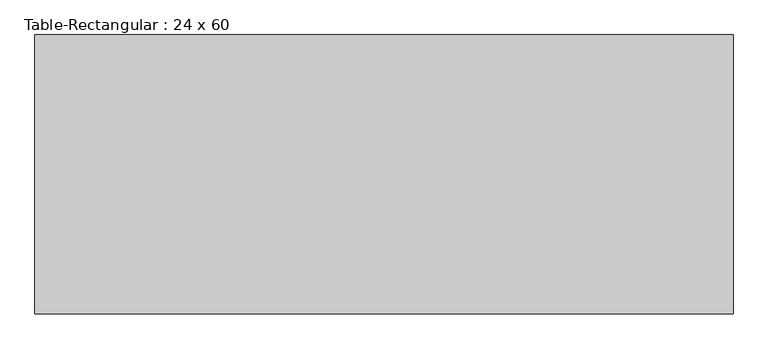
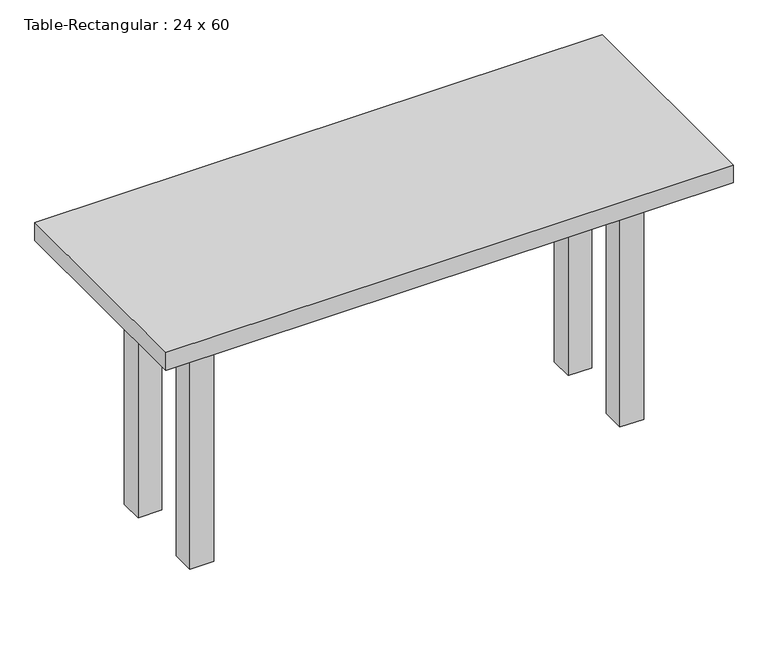
"""IFC4 building model written with IfcOpenShell, lengths in millimetres: furniture geometry, Table-Rectangular : 24 x 60."""

from ifc_helpers import new_model, si_unit, frame, origin, origin_with_axes, place, context, project, spatial, polyline, outline, extrude, source, transform, mapped, element, save


def table_rectangular_24_x_60_3e3a90ab(model_context):
    return source(origin(), model_context, "Body", "SweptSolid", [
        extrude(outline(polyline([(546.1, 114.3), (546.1, 88.9), (-546.1, 88.9), (-546.1, 114.3), (546.1, 114.3)])), frame((0.0, 0.0, 609.6), z_axis=(0.0, 0.0, 1.0), x_axis=(1.0, 0.0, 0.0)), (0.0, 0.0, 1.0), 101.6),
        extrude(outline(polyline([(546.1, -114.3), (-546.1, -114.3), (-546.1, -88.9), (546.1, -88.9), (546.1, -114.3)])), frame((0.0, 0.0, 609.6), z_axis=(0.0, 0.0, 1.0), x_axis=(1.0, 0.0, 0.0)), (0.0, 0.0, 1.0), 101.6),
        extrude(outline(polyline([(-558.8, -88.9), (-584.2, -88.9), (-584.2, 88.9), (-558.8, 88.9), (-558.8, -88.9)])), frame((0.0, 0.0, 609.6), z_axis=(0.0, 0.0, 1.0), x_axis=(1.0, 0.0, 0.0)), (0.0, 0.0, 1.0), 101.6),
        extrude(outline(polyline([(558.8, -88.9), (558.8, 88.9), (584.2, 88.9), (584.2, -88.9), (558.8, -88.9)])), frame((0.0, 0.0, 609.6), z_axis=(0.0, 0.0, 1.0), x_axis=(1.0, 0.0, 0.0)), (0.0, 0.0, 1.0), 101.6),
        extrude(outline(polyline([(762.0, 304.8), (762.0, -304.8), (-762.0, -304.8), (-762.0, 304.8), (762.0, 304.8)])), frame((0.0, 0.0, 711.2), z_axis=(0.0, 0.0, 1.0), x_axis=(1.0, 0.0, 0.0)), (0.0, 0.0, 1.0), 50.8),
        extrude(outline(polyline([(-546.1, 152.4), (-546.1, 88.9), (-609.6, 88.9), (-609.6, 152.4), (-546.1, 152.4)])), origin_with_axes(), (0.0, 0.0, 1.0), 711.2),
        extrude(outline(polyline([(546.1, 152.4), (609.6, 152.4), (609.6, 88.9), (546.1, 88.9), (546.1, 152.4)])), origin_with_axes(), (0.0, 0.0, 1.0), 711.2),
        extrude(outline(polyline([(-546.1, -152.4), (-609.6, -152.4), (-609.6, -88.9), (-546.1, -88.9), (-546.1, -152.4)])), origin_with_axes(), (0.0, 0.0, 1.0), 711.2),
        extrude(outline(polyline([(546.1, -152.4), (546.1, -88.9), (609.6, -88.9), (609.6, -152.4), (546.1, -152.4)])), origin_with_axes(), (0.0, 0.0, 1.0), 711.2),
    ])


if __name__ == "__main__":
    model = new_model("IFC4")
    model_context = context("Model", 3, world=origin())
    ifc_project = project(units=[si_unit("LENGTHUNIT", "METRE", prefix="MILLI")], contexts=[model_context])
    site = spatial("IfcSite", under=ifc_project)
    building = spatial("IfcBuilding", under=site)
    placement = place(None, origin())
    table_rectangular_24_x_60_shape = table_rectangular_24_x_60_3e3a90ab(model_context)
    element("IfcFurniture", 1, ObjectType="Table-Rectangular : 24 x 60", at=placement, inside=building, context=model_context, shape_type="MappedRepresentation", body=[
        mapped(table_rectangular_24_x_60_shape, transform((0.0, 0.0, 0.0), x_axis=(1.0, 0.0, 0.0), y_axis=(0.0, 1.0, 0.0), z_axis=(0.0, 0.0, 1.0))),
    ])
    save(model, "model.ifc")

# Revit data of these elements
# Type "Table-Rectangular : 24 x 60"
#   Assembly Code = "E2020200"
#   Height = 2' - 6"
#   Length = 5' - 0"
#   Width = 2' - 0"
#   Base Material = Wood - Birch
#   Top Material = Wood - Birch
#   Default Elevation = 0
# Element 1 (IfcFurniture, "Table-Rectangular : 24 x 60")
#   Materials on its faces: "Wood - Birch"
# Materials
#   "Wood - Birch": class "Unassigned", colour RGB 224 178 126, transparency 0
